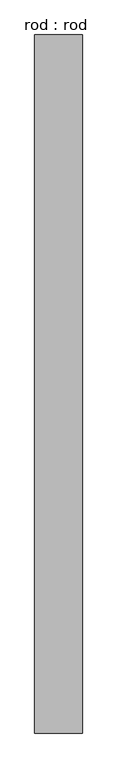
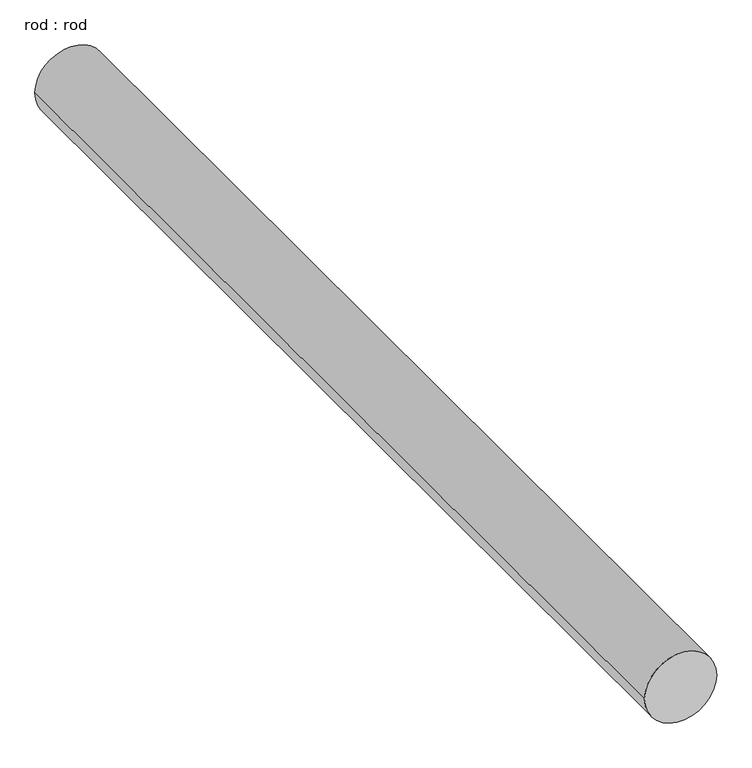
"""IFC4 building model written with IfcOpenShell, lengths in millimetres: proxy geometry, rod : rod."""

from ifc_helpers import new_model, si_unit, point, frame, frame_2d, origin, place, context, project, spatial, circle_curve, trimmed, segment, composite_curve, outline, extrude, source, transform, mapped, element, save


def rod_rod_78ba7e92(model_context):
    return source(origin(), model_context, "Body", "SweptSolid", [
        extrude(outline(composite_curve([segment(trimmed(circle_curve(frame_2d((0.0108462, 0.0)), 200.0), [point((0.0108462, 200.0))], [point((0.0108462, -200.0))], False, "CARTESIAN"), True, "CONTINUOUS"), segment(trimmed(circle_curve(frame_2d((0.0108462, 0.0)), 200.0), [point((0.0108462, -200.0))], [point((0.0108462, 200.0))], False, "CARTESIAN"), True, "CONTINUOUS")], self_intersect=False)), frame((0.0, 1162.1940545, 0.0), z_axis=(0.0, 1.0, 0.0), x_axis=(0.0, 0.0, 1.0)), (0.0, 0.0, 1.0), 5861.0691218),
    ])


if __name__ == "__main__":
    model = new_model("IFC4")
    model_context = context("Model", 3, world=origin())
    ifc_project = project(units=[si_unit("LENGTHUNIT", "METRE", prefix="MILLI")], contexts=[model_context])
    site = spatial("IfcSite", under=ifc_project)
    building = spatial("IfcBuilding", under=site)
    placement = place(None, origin())
    rod_rod_shape = rod_rod_78ba7e92(model_context)
    element("IfcBuildingElementProxy", 1, Name="rod : rod", ObjectType="rod : rod", at=placement, inside=building, context=model_context, shape_type="MappedRepresentation", body=[
        mapped(rod_rod_shape, transform((0.0, 0.0, 0.0), x_axis=(1.0, 0.0, 0.0), y_axis=(0.0, 1.0, 0.0), z_axis=(0.0, 0.0, 1.0))),
    ])
    save(model, "model.ifc")

# Revit data of these elements
# Type "rod : rod"
#   Default Elevation = 0
